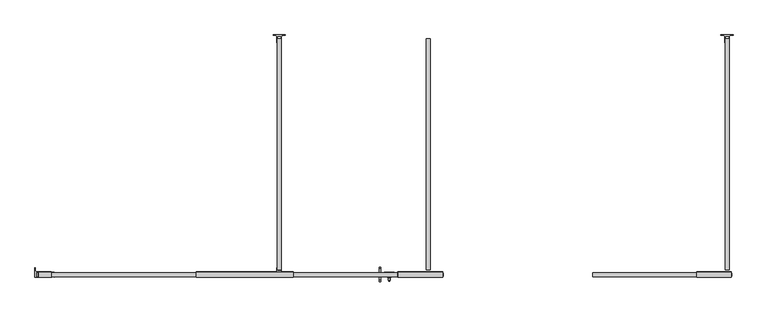
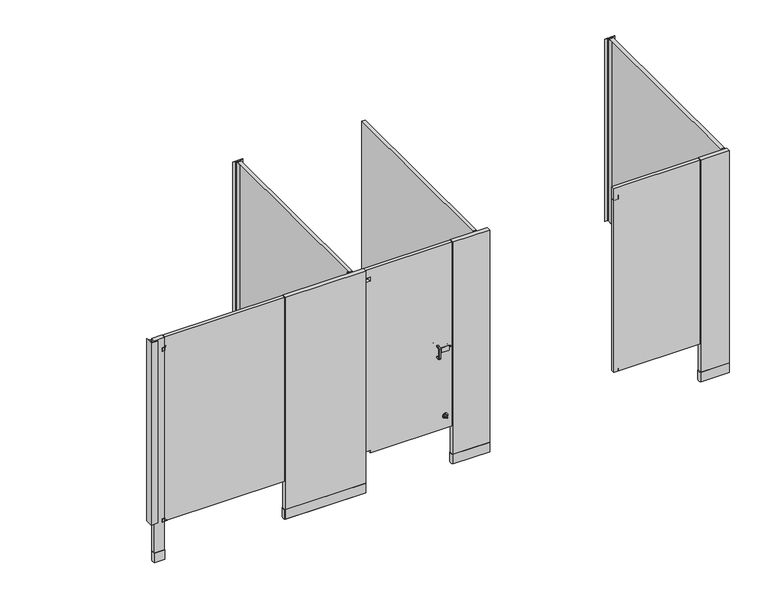
"""IFC4 building model written with IfcOpenShell, lengths in millimetres: proxy geometry, Partition-Floor_Braced-Bradley_Corp-St_Stl-ADA-N_Stalls : ADA (optional) + n Standard Stalls."""

from ifc_helpers import new_model, si_unit, point, frame, frame_2d, origin, origin_with_axes, place, context, project, spatial, polyline, circle_curve, ellipse_curve, trimmed, segment, composite_curve, outline, extrude, source, transform, mapped, element, save
from ifc_brep_helpers import plane_surface, cylinder_surface, revolved_surface, advanced_brep


def specialty_equipment_511efb68(model_context):
    return source(origin(), model_context, "Body", "SolidModel", [
        extrude(outline(composite_curve([segment(polyline([(4584.7002547, 3.175), (4584.7002547, 0.635), (4568.1902547, 0.635)]), True, "CONTINUOUS"), segment(trimmed(circle_curve(frame_2d((4568.1902547, -5.715)), 6.35), [point((4568.1902547, 0.635))], [point((4561.8402547, -5.715))], True, "CARTESIAN"), True, "CONTINUOUS"), segment(polyline([(4561.8402547, -5.715), (4561.8402547, -47.625), (4559.3002547, -47.625), (4559.3002547, -3.7728188), (4533.9002547, -3.7728188), (4533.9002547, -47.625), (4531.3602547, -47.625), (4531.3602547, -5.715)]), True, "CONTINUOUS"), segment(trimmed(circle_curve(frame_2d((4525.0102547, -5.715)), 6.35), [point((4531.3602547, -5.715))], [point((4525.0102547, 0.635))], True, "CARTESIAN"), True, "CONTINUOUS"), segment(polyline([(4525.0102547, 0.635), (4508.5002547, 0.635), (4508.5002547, 3.175), (4584.7002547, 3.175)]), True, "CONTINUOUS")], self_intersect=False)), frame((0.0, 0.0, 311.15), z_axis=(0.0, 0.0, 1.0), x_axis=(1.0, 0.0, 0.0)), (0.0, 0.0, 1.0), 1460.5),
        extrude(outline(composite_curve([segment(trimmed(circle_curve(frame_2d((301.9554547, -1504.95)), 2.54), [point((301.9554547, -1507.49))], [point((301.9554547, -1502.41))], False, "CARTESIAN"), True, "CONTINUOUS"), segment(trimmed(circle_curve(frame_2d((301.9554547, -1504.95)), 2.54), [point((301.9554547, -1502.41))], [point((301.9554547, -1507.49))], False, "CARTESIAN"), True, "CONTINUOUS")], self_intersect=False)), frame((0.0, 0.0, 304.8), z_axis=(0.0, 0.0, 1.0), x_axis=(1.0, 0.0, 0.0)), (0.0, 0.0, 1.0), 25.4),
        extrude(outline(composite_curve([segment(polyline([(292.1002547, -1489.71), (313.6902547, -1489.075), (323.8502547, -1497.33)]), True, "CONTINUOUS"), segment(trimmed(circle_curve(frame_2d((320.0402547, -1504.95)), 8.519419), [point((323.8502547, -1497.33))], [point((323.8502547, -1512.57))], False, "CARTESIAN"), True, "CONTINUOUS"), segment(polyline([(323.8502547, -1512.57), (313.6902547, -1520.825), (292.1002547, -1520.19), (292.1002547, -1489.71)]), True, "CONTINUOUS")], self_intersect=False)), frame((0.0, 0.0, 304.8), z_axis=(0.0, 0.0, 1.0), x_axis=(1.0, 0.0, 0.0)), (0.0, 0.0, 1.0), 3.81),
        extrude(outline(composite_curve([segment(polyline([(273.0502547, -1486.535), (292.1002547, -1486.535)]), True, "CONTINUOUS"), segment(trimmed(circle_curve(frame_2d((292.1002547, -1489.075)), 2.54), [point((292.1002547, -1486.535))], [point((294.6402547, -1489.075))], False, "CARTESIAN"), True, "CONTINUOUS"), segment(trimmed(circle_curve(frame_2d((186.8397496, -1504.95)), 108.9631338), [point((294.6402547, -1489.075))], [point((294.6402547, -1520.825))], False, "CARTESIAN"), True, "CONTINUOUS"), segment(trimmed(circle_curve(frame_2d((292.1002547, -1520.825)), 2.54), [point((294.6402547, -1520.825))], [point((292.1002547, -1523.365))], False, "CARTESIAN"), True, "CONTINUOUS"), segment(polyline([(292.1002547, -1523.365), (273.0502547, -1523.365), (273.0502547, -1486.535)]), True, "CONTINUOUS")], self_intersect=False)), frame((0.0, 0.0, 304.8), z_axis=(0.0, 0.0, 1.0), x_axis=(1.0, 0.0, 0.0)), (0.0, 0.0, 1.0), 25.4),
        extrude(outline(composite_curve([segment(trimmed(circle_curve(frame_2d((301.9554547, -1504.95)), 2.54), [point((301.9554547, -1507.49))], [point((301.9554547, -1502.41))], False, "CARTESIAN"), True, "CONTINUOUS"), segment(trimmed(circle_curve(frame_2d((301.9554547, -1504.95)), 2.54), [point((301.9554547, -1502.41))], [point((301.9554547, -1507.49))], False, "CARTESIAN"), True, "CONTINUOUS")], self_intersect=False)), frame((0.0, 0.0, 1676.4), z_axis=(0.0, 0.0, 1.0), x_axis=(1.0, 0.0, 0.0)), (0.0, 0.0, 1.0), 25.4),
        extrude(outline(composite_curve([segment(polyline([(296.8754547, -1520.825), (292.1002547, -1520.19), (292.1002547, -1489.71), (296.8754547, -1489.075), (307.0354547, -1497.33)]), True, "CONTINUOUS"), segment(trimmed(circle_curve(frame_2d((303.2254547, -1504.95)), 8.519419), [point((307.0354547, -1497.33))], [point((307.0354547, -1512.57))], False, "CARTESIAN"), True, "CONTINUOUS"), segment(polyline([(307.0354547, -1512.57), (296.8754547, -1520.825)]), True, "CONTINUOUS")], self_intersect=False)), frame((0.0, 0.0, 1697.99), z_axis=(0.0, 0.0, 1.0), x_axis=(1.0, 0.0, 0.0)), (0.0, 0.0, 1.0), 3.81),
        extrude(outline(composite_curve([segment(polyline([(273.0502547, -1486.535), (292.1002547, -1486.535)]), True, "CONTINUOUS"), segment(trimmed(circle_curve(frame_2d((292.1002547, -1489.075)), 2.54), [point((292.1002547, -1486.535))], [point((294.6402547, -1489.075))], False, "CARTESIAN"), True, "CONTINUOUS"), segment(trimmed(circle_curve(frame_2d((186.8397496, -1504.95)), 108.9631338), [point((294.6402547, -1489.075))], [point((294.6402547, -1520.825))], False, "CARTESIAN"), True, "CONTINUOUS"), segment(trimmed(circle_curve(frame_2d((292.1002547, -1520.825)), 2.54), [point((294.6402547, -1520.825))], [point((292.1002547, -1523.365))], False, "CARTESIAN"), True, "CONTINUOUS"), segment(polyline([(292.1002547, -1523.365), (273.0502547, -1523.365), (273.0502547, -1486.535)]), True, "CONTINUOUS")], self_intersect=False)), frame((0.0, 0.0, 1676.4), z_axis=(0.0, 0.0, 1.0), x_axis=(1.0, 0.0, 0.0)), (0.0, 0.0, 1.0), 25.4),
        extrude(outline(composite_curve([segment(polyline([(190.5002547, -1463.675), (193.0402547, -1463.675), (193.0402547, -1480.185)]), True, "CONTINUOUS"), segment(trimmed(circle_curve(frame_2d((199.3902547, -1480.185)), 6.35), [point((193.0402547, -1480.185))], [point((199.3902547, -1486.535))], True, "CARTESIAN"), True, "CONTINUOUS"), segment(polyline([(199.3902547, -1486.535), (241.3002547, -1486.535), (241.3002547, -1489.075), (197.4480735, -1489.075), (197.4480735, -1520.825), (241.3002547, -1520.825), (241.3002547, -1523.365), (190.5002547, -1523.365), (190.5002547, -1463.675)]), True, "CONTINUOUS")], self_intersect=False)), frame((0.0, 0.0, 311.15), z_axis=(0.0, 0.0, 1.0), x_axis=(1.0, 0.0, 0.0)), (0.0, 0.0, 1.0), 1460.5),
        extrude(outline(polyline([(1711.9602547, -1489.075), (1711.9602547, -1463.675), (1714.5002547, -1463.675), (1714.5002547, -1482.1271812), (1739.9002547, -1482.1271812), (1739.9002547, -1463.675), (1742.4402547, -1463.675), (1742.4402547, -1489.075), (1711.9602547, -1489.075)])), frame((0.0, 0.0, 311.15), z_axis=(0.0, 0.0, 1.0), x_axis=(1.0, 0.0, 0.0)), (0.0, 0.0, 1.0), 1460.5),
        extrude(outline(composite_curve([segment(polyline([(1765.3002547, 3.175), (1765.3002547, 0.635), (1748.7902547, 0.635)]), True, "CONTINUOUS"), segment(trimmed(circle_curve(frame_2d((1748.7902547, -5.715)), 6.35), [point((1748.7902547, 0.635))], [point((1742.4402547, -5.715))], True, "CARTESIAN"), True, "CONTINUOUS"), segment(polyline([(1742.4402547, -5.715), (1742.4402547, -47.625), (1739.9002547, -47.625), (1739.9002547, -3.7728188), (1714.5002547, -3.7728188), (1714.5002547, -47.625), (1711.9602547, -47.625), (1711.9602547, -5.715)]), True, "CONTINUOUS"), segment(trimmed(circle_curve(frame_2d((1705.6102547, -5.715)), 6.35), [point((1711.9602547, -5.715))], [point((1705.6102547, 0.635))], True, "CARTESIAN"), True, "CONTINUOUS"), segment(polyline([(1705.6102547, 0.635), (1689.1002547, 0.635), (1689.1002547, 3.175), (1765.3002547, 3.175)]), True, "CONTINUOUS")], self_intersect=False)), frame((0.0, 0.0, 311.15), z_axis=(0.0, 0.0, 1.0), x_axis=(1.0, 0.0, 0.0)), (0.0, 0.0, 1.0), 1460.5),
        extrude(outline(composite_curve([segment(polyline([(214.3127547, -1487.4875), (293.6891337, -1487.4875)]), True, "CONTINUOUS"), segment(trimmed(circle_curve(frame_2d((237.900102, -1504.95)), 58.4581471), [point((293.6891337, -1487.4875))], [point((293.6891337, -1522.4125))], False, "CARTESIAN"), True, "CONTINUOUS"), segment(polyline([(293.6891337, -1522.4125), (214.3127547, -1522.4125)]), True, "CONTINUOUS"), segment(trimmed(circle_curve(frame_2d((270.1017864, -1504.95)), 58.4581471), [point((214.3127547, -1522.4125))], [point((214.3127547, -1487.4875))], False, "CARTESIAN"), True, "CONTINUOUS")], self_intersect=False)), origin_with_axes(), (0.0, 0.0, 1.0), 76.2),
        extrude(outline(composite_curve([segment(polyline([(1204.9127547, -1487.4875), (1817.6891337, -1487.4875)]), True, "CONTINUOUS"), segment(trimmed(circle_curve(frame_2d((1761.900102, -1504.95)), 58.4581471), [point((1817.6891337, -1487.4875))], [point((1817.6891337, -1522.4125))], False, "CARTESIAN"), True, "CONTINUOUS"), segment(polyline([(1817.6891337, -1522.4125), (1204.9127547, -1522.4125)]), True, "CONTINUOUS"), segment(trimmed(circle_curve(frame_2d((1260.7017864, -1504.95)), 58.4581471), [point((1204.9127547, -1522.4125))], [point((1204.9127547, -1487.4875))], False, "CARTESIAN"), True, "CONTINUOUS")], self_intersect=False)), origin_with_axes(), (0.0, 0.0, 1.0), 76.2),
        extrude(outline(composite_curve([segment(polyline([(4354.5127547, -1487.4875), (4573.5891337, -1487.4875)]), True, "CONTINUOUS"), segment(trimmed(circle_curve(frame_2d((4517.800102, -1504.95)), 58.4581471), [point((4573.5891337, -1487.4875))], [point((4573.5891337, -1522.4125))], False, "CARTESIAN"), True, "CONTINUOUS"), segment(polyline([(4573.5891337, -1522.4125), (4354.5127547, -1522.4125)]), True, "CONTINUOUS"), segment(trimmed(circle_curve(frame_2d((4410.3017864, -1504.95)), 58.4581471), [point((4354.5127547, -1522.4125))], [point((4354.5127547, -1487.4875))], False, "CARTESIAN"), True, "CONTINUOUS")], self_intersect=False)), origin_with_axes(), (0.0, 0.0, 1.0), 76.2),
        extrude(outline(composite_curve([segment(trimmed(circle_curve(frame_2d((-1469.3891724, 977.9)), 10.16), [point((-1469.3891724, 988.06))], [point((-1459.2291724, 977.9))], False, "CARTESIAN"), True, "CONTINUOUS"), segment(polyline([(-1459.2291724, 977.9), (-1459.2291724, 901.7)]), True, "CONTINUOUS"), segment(trimmed(circle_curve(frame_2d((-1469.3891724, 901.7)), 10.16), [point((-1459.2291724, 901.7))], [point((-1469.3891724, 891.54))], False, "CARTESIAN"), True, "CONTINUOUS"), segment(polyline([(-1469.3891724, 891.54), (-1492.2491724, 891.54), (-1492.2491724, 901.7), (-1469.3891724, 901.7)]), True, "CONTINUOUS"), segment(trimmed(circle_curve(frame_2d((-1469.3891724, 904.24)), 2.54), [point((-1469.3891724, 901.7))], [point((-1466.8491724, 904.24))], True, "CARTESIAN"), True, "CONTINUOUS"), segment(polyline([(-1466.8491724, 904.24), (-1466.8491724, 975.36)]), True, "CONTINUOUS"), segment(trimmed(circle_curve(frame_2d((-1469.3891724, 975.36)), 2.54), [point((-1466.8491724, 975.36))], [point((-1469.3891724, 977.9))], True, "CARTESIAN"), True, "CONTINUOUS"), segment(polyline([(-1469.3891724, 977.9), (-1492.2491724, 977.9), (-1492.2491724, 988.06), (-1469.3891724, 988.06)]), True, "CONTINUOUS")], self_intersect=False)), frame((2356.5228738, 0.0, 0.0), z_axis=(1.0, 0.0, 0.0), x_axis=(0.0, 1.0, 0.0)), (0.0, 0.0, 1.0), 11.4113578),
        extrude(outline(composite_curve([segment(polyline([(-1540.51, 988.06), (-1517.65, 988.06), (-1517.65, 977.9), (-1540.51, 977.9)]), True, "CONTINUOUS"), segment(trimmed(circle_curve(frame_2d((-1540.51, 975.36)), 2.54), [point((-1540.51, 977.9))], [point((-1543.05, 975.36))], True, "CARTESIAN"), True, "CONTINUOUS"), segment(polyline([(-1543.05, 975.36), (-1543.05, 904.24)]), True, "CONTINUOUS"), segment(trimmed(circle_curve(frame_2d((-1540.51, 904.24)), 2.54), [point((-1543.05, 904.24))], [point((-1540.51, 901.7))], True, "CARTESIAN"), True, "CONTINUOUS"), segment(polyline([(-1540.51, 901.7), (-1517.65, 901.7), (-1517.65, 891.54), (-1540.51, 891.54)]), True, "CONTINUOUS"), segment(trimmed(circle_curve(frame_2d((-1540.51, 901.7)), 10.16), [point((-1540.51, 891.54))], [point((-1550.67, 901.7))], False, "CARTESIAN"), True, "CONTINUOUS"), segment(polyline([(-1550.67, 901.7), (-1550.67, 977.9)]), True, "CONTINUOUS"), segment(trimmed(circle_curve(frame_2d((-1540.51, 977.9)), 10.16), [point((-1550.67, 977.9))], [point((-1540.51, 988.06))], False, "CARTESIAN"), True, "CONTINUOUS")], self_intersect=False)), frame((2356.5228738, 0.0, 0.0), z_axis=(1.0, 0.0, 0.0), x_axis=(0.0, 1.0, 0.0)), (0.0, 0.0, 1.0), 11.4113578),
        extrude(outline(composite_curve([segment(trimmed(circle_curve(frame_2d((406.4, 2420.9250547)), 3.4532283), [point((402.9467717, 2420.9250547))], [point((409.8532283, 2420.9250547))], False, "CARTESIAN"), True, "CONTINUOUS"), segment(trimmed(circle_curve(frame_2d((406.4, 2420.9250547)), 3.4532283), [point((409.8532283, 2420.9250547))], [point((402.9467717, 2420.9250547))], False, "CARTESIAN"), True, "CONTINUOUS")], self_intersect=False)), frame((0.0, -1548.13, 0.0), z_axis=(0.0, 1.0, 0.0), x_axis=(0.0, 0.0, 1.0)), (0.0, 0.0, 1.0), 7.62),
        advanced_brep(
        [(2420.9250547, -1517.65, 406.4), (2401.8750547, -1517.65, 406.4), (2439.9750547, -1517.65, 406.4), (2426.0050547, -1540.51, 406.4), (2415.8450547, -1540.51, 406.4), (2420.9250547, -1540.51, 406.4), (2426.0050547, -1525.27, 406.4), (2415.8450547, -1525.27, 406.4), (2431.0850547, -1520.19, 406.4), (2410.7650547, -1520.19, 406.4), (2439.9750547, -1520.19, 406.4), (2401.8750547, -1520.19, 406.4)],
        [
            (0, 1),
            (1, 2, circle_curve(frame((2420.9250547, -1517.65, 406.4), z_axis=(0.0, 1.0, 0.0), x_axis=(-1.0, 0.0, 0.0)), 19.05)),
            (2, 0),
            (2, 1, circle_curve(frame((2420.9250547, -1517.65, 406.4), z_axis=(0.0, 1.0, 0.0), x_axis=(-1.0, 0.0, 0.0)), 19.05)),
            (3, 4, circle_curve(frame((2420.9250547, -1540.51, 406.4), z_axis=(0.0, -1.0, 0.0), x_axis=(-1.0, 0.0, 0.0)), 5.08)),
            (4, 5),
            (5, 3),
            (4, 3, circle_curve(frame((2420.9250547, -1540.51, 406.4), z_axis=(0.0, -1.0, 0.0), x_axis=(-1.0, 0.0, 0.0)), 5.08)),
            (6, 7, circle_curve(frame((2420.9250547, -1525.27, 406.4), z_axis=(0.0, -1.0, 0.0), x_axis=(-1.0, 0.0, 0.0)), 5.08)),
            (7, 4),
            (3, 6),
            (7, 6, circle_curve(frame((2420.9250547, -1525.27, 406.4), z_axis=(0.0, -1.0, 0.0), x_axis=(-1.0, 0.0, 0.0)), 5.08)),
            (8, 9, circle_curve(frame((2420.9250547, -1520.19, 406.4), z_axis=(0.0, -1.0, 0.0), x_axis=(-1.0, 0.0, 0.0)), 10.16)),
            (9, 7, circle_curve(frame((2415.8450547, -1520.19, 406.4), z_axis=(0.0, 0.0, 1.0), x_axis=(0.0, -1.0, 0.0)), 5.08)),
            (6, 8, circle_curve(frame((2426.0050547, -1520.19, 406.4), z_axis=(0.0, 0.0, 1.0), x_axis=(0.0, -1.0, 0.0)), 5.08)),
            (9, 8, circle_curve(frame((2420.9250547, -1520.19, 406.4), z_axis=(0.0, -1.0, 0.0), x_axis=(-1.0, 0.0, 0.0)), 10.16)),
            (10, 11, circle_curve(frame((2420.9250547, -1520.19, 406.4), z_axis=(0.0, -1.0, 0.0), x_axis=(-1.0, 0.0, 0.0)), 19.05)),
            (11, 9),
            (8, 10),
            (11, 10, circle_curve(frame((2420.9250547, -1520.19, 406.4), z_axis=(0.0, -1.0, 0.0), x_axis=(-1.0, 0.0, 0.0)), 19.05)),
            (1, 11),
            (10, 2),
        ],
        [
            plane_surface(frame((2420.9250547, -1517.65, 406.4), z_axis=(0.0, 1.0, 0.0), x_axis=(-1.0, 0.0, 0.0))),
            plane_surface(frame((2420.9250547, -1540.51, 406.4), z_axis=(0.0, -1.0, 0.0), x_axis=(-1.0, 0.0, 0.0))),
            cylinder_surface(frame((2420.9250547, -1561.6297247, 406.4), z_axis=(0.0, 1.0, 0.0), x_axis=(-1.0, 0.0, 0.0)), 5.08),
            revolved_surface(trimmed(ellipse_curve(frame((2415.8450547, -1520.19, 406.4), z_axis=(0.0, 0.0, -1.0), x_axis=(0.0, -1.0, 0.0)), 5.08, 5.08), [point((2415.8450547, -1525.27, 406.4))], [point((2410.7650547, -1520.19, 406.4))], True, "CARTESIAN"), (2420.9250547, -1561.6297247, 406.4), (0.0, 1.0, 0.0)),
            plane_surface(frame((2420.9250547, -1520.19, 406.4), z_axis=(0.0, -1.0, 0.0), x_axis=(-1.0, 0.0, 0.0))),
            cylinder_surface(frame((2420.9250547, -1561.6297247, 406.4), z_axis=(0.0, 1.0, 0.0), x_axis=(-1.0, 0.0, 0.0)), 19.05),
        ],
        [
            (0, [[1, 2, 3]]),
            (0, [[-3, 4, -1]]),
            (1, [[5, 6, 7]]),
            (1, [[8, -7, -6]]),
            (2, [[9, 10, -5, 11]]),
            (2, [[12, -11, -8, -10]]),
            (3, [[13, 14, -9, 15]]),
            (3, [[16, -15, -12, -14]]),
            (4, [[17, 18, -13, 19]]),
            (4, [[20, -19, -16, -18]]),
            (5, [[-2, 21, -17, 22]]),
            (5, [[-4, -22, -20, -21]]),
        ],
    ),
        advanced_brep(
        [(2465.3750547, -1499.87, 939.8), (2465.3750547, -1510.03, 939.8), (2482.8502547, -1510.03, 939.8), (2482.8502547, -1499.87, 939.8), (2465.3750547, -1504.95, 939.8), (2482.8502547, -1504.95, 939.8)],
        [
            (0, 1, circle_curve(frame((2465.3750547, -1504.95, 939.8), z_axis=(1.0, 0.0, 0.0), x_axis=(0.0, -1.0, 0.0)), 5.08)),
            (1, 2),
            (2, 3, circle_curve(frame((2482.8502547, -1504.95, 939.8), z_axis=(-1.0, 0.0, 0.0), x_axis=(0.0, -1.0, 0.0)), 5.08)),
            (3, 0),
            (1, 0, circle_curve(frame((2465.3750547, -1504.95, 939.8), z_axis=(1.0, 0.0, 0.0), x_axis=(0.0, -1.0, 0.0)), 5.08)),
            (3, 2, circle_curve(frame((2482.8502547, -1504.95, 939.8), z_axis=(-1.0, 0.0, 0.0), x_axis=(0.0, -1.0, 0.0)), 5.08)),
            (4, 1),
            (0, 4),
            (2, 5),
            (5, 3),
        ],
        [
            cylinder_surface(frame((2482.8502547, -1504.95, 939.8), z_axis=(-1.0, 0.0, 0.0), x_axis=(0.0, -1.0, 0.0)), 5.08),
            plane_surface(frame((2465.3750547, -1504.95, 939.8), z_axis=(-1.0, 0.0, 0.0), x_axis=(0.0, -1.0, 0.0))),
            plane_surface(frame((2482.8502547, -1504.95, 939.8), z_axis=(1.0, 0.0, 0.0), x_axis=(0.0, -1.0, 0.0))),
        ],
        [
            (0, [[1, 2, 3, 4]]),
            (0, [[5, -4, 6, -2]]),
            (1, [[7, -1, 8]]),
            (1, [[-8, -5, -7]]),
            (2, [[-3, 9, 10]]),
            (2, [[-6, -10, -9]]),
        ],
    ),
        extrude(outline(composite_curve([segment(trimmed(circle_curve(frame_2d((926.0058992, 2394.4309539)), 5.2558992), [point((926.0058992, 2389.1750547))], [point((920.75, 2394.4309539))], False, "CARTESIAN"), True, "CONTINUOUS"), segment(polyline([(920.75, 2394.4309539), (920.75, 2447.4191555)]), True, "CONTINUOUS"), segment(trimmed(circle_curve(frame_2d((926.0058992, 2447.4191555)), 5.2558992), [point((920.75, 2447.4191555))], [point((926.0058992, 2452.6750547))], False, "CARTESIAN"), True, "CONTINUOUS"), segment(polyline([(926.0058992, 2452.6750547), (953.5941008, 2452.6750547)]), True, "CONTINUOUS"), segment(trimmed(circle_curve(frame_2d((953.5941008, 2447.4191555)), 5.2558992), [point((953.5941008, 2452.6750547))], [point((958.85, 2447.4191555))], False, "CARTESIAN"), True, "CONTINUOUS"), segment(polyline([(958.85, 2447.4191555), (958.85, 2394.4309539)]), True, "CONTINUOUS"), segment(trimmed(circle_curve(frame_2d((953.5941008, 2394.4309539)), 5.2558992), [point((958.85, 2394.4309539))], [point((953.5941008, 2389.1750547))], False, "CARTESIAN"), True, "CONTINUOUS"), segment(polyline([(953.5941008, 2389.1750547), (926.0058992, 2389.1750547)]), True, "CONTINUOUS")], self_intersect=False)), frame((0.0, -1519.555, 0.0), z_axis=(0.0, 1.0, 0.0), x_axis=(0.0, 0.0, 1.0)), (0.0, 0.0, 1.0), 29.21),
        extrude(outline(composite_curve([segment(polyline([(2474.9127547, -1487.4875), (2757.4891337, -1487.4875)]), True, "CONTINUOUS"), segment(trimmed(circle_curve(frame_2d((2701.700102, -1504.95)), 58.4581471), [point((2757.4891337, -1487.4875))], [point((2757.4891337, -1522.4125))], False, "CARTESIAN"), True, "CONTINUOUS"), segment(polyline([(2757.4891337, -1522.4125), (2474.9127547, -1522.4125)]), True, "CONTINUOUS"), segment(trimmed(circle_curve(frame_2d((2530.7017864, -1504.95)), 58.4581471), [point((2474.9127547, -1522.4125))], [point((2474.9127547, -1487.4875))], False, "CARTESIAN"), True, "CONTINUOUS")], self_intersect=False)), origin_with_axes(), (0.0, 0.0, 1.0), 76.2),
        extrude(outline(polyline([(2679.7002547, -22.225), (2679.7002547, -1476.375), (2654.3002547, -1476.375), (2654.3002547, -22.225), (2679.7002547, -22.225)])), frame((0.0, 0.0, 304.8), z_axis=(0.0, 0.0, 1.0), x_axis=(1.0, 0.0, 0.0)), (0.0, 0.0, 1.0), 1473.2),
        extrude(outline(polyline([(2476.5002547, -1489.075), (2755.9002547, -1489.075), (2755.9002547, -1520.825), (2476.5002547, -1520.825), (2476.5002547, -1489.075)])), origin_with_axes(), (0.0, 0.0, 1.0), 1778.0),
        extrude(outline(polyline([(1778.0, 2471.7250547), (1778.0, 1820.8754547), (1714.5, 1820.8754547), (1714.5, 1852.6254547), (1682.75, 1852.6254547), (1682.75, 1820.8754547), (323.85, 1820.8754547), (323.85, 1852.6254547), (304.8, 1852.6254547), (304.8, 2471.7250547), (1778.0, 2471.7250547)])), frame((0.0, -1517.65, 0.0), z_axis=(0.0, 1.0, 0.0), x_axis=(0.0, 0.0, 1.0)), (0.0, 0.0, 1.0), 25.4),
        extrude(outline(polyline([(1201.7250547, -1517.65), (296.8754547, -1517.65), (296.8754547, -1492.25), (1201.7250547, -1492.25), (1201.7250547, -1517.65)])), frame((0.0, 0.0, 304.8), z_axis=(0.0, 0.0, 1.0), x_axis=(1.0, 0.0, 0.0)), (0.0, 0.0, 1.0), 1473.2),
        extrude(outline(polyline([(4351.3250547, -1517.65), (3700.4754547, -1517.65), (3700.4754547, -1492.25), (4351.3250547, -1492.25), (4351.3250547, -1517.65)])), frame((0.0, 0.0, 304.8), z_axis=(0.0, 0.0, 1.0), x_axis=(1.0, 0.0, 0.0)), (0.0, 0.0, 1.0), 1473.2),
        extrude(outline(polyline([(1778.0, 4351.3250547), (1778.0, 3700.4754547), (1714.5, 3700.4754547), (1714.5, 3732.2254547), (1682.75, 3732.2254547), (1682.75, 3700.4754547), (323.85, 3700.4754547), (323.85, 3732.2254547), (304.8, 3732.2254547), (304.8, 4351.3250547), (1778.0, 4351.3250547)])), frame((0.0, -1517.65, 0.0), z_axis=(0.0, 1.0, 0.0), x_axis=(0.0, 0.0, 1.0)), (0.0, 0.0, 1.0), 25.4),
        extrude(outline(polyline([(1778.0, 1201.7250547), (1778.0, 296.8754547), (1714.5, 296.8754547), (1714.5, 328.6254547), (1682.75, 328.6254547), (1682.75, 296.8754547), (323.85, 296.8754547), (323.85, 328.6254547), (304.8, 328.6254547), (304.8, 1201.7250547), (1778.0, 1201.7250547)])), frame((0.0, -1517.65, 0.0), z_axis=(0.0, 1.0, 0.0), x_axis=(0.0, 0.0, 1.0)), (0.0, 0.0, 1.0), 25.4),
        extrude(outline(polyline([(4356.1002547, -1489.075), (4572.0002547, -1489.075), (4572.0002547, -1520.825), (4356.1002547, -1520.825), (4356.1002547, -1489.075)])), origin_with_axes(), (0.0, 0.0, 1.0), 1778.0),
        extrude(outline(polyline([(1206.5002547, -1489.075), (1816.1002547, -1489.075), (1816.1002547, -1520.825), (1206.5002547, -1520.825), (1206.5002547, -1489.075)])), origin_with_axes(), (0.0, 0.0, 1.0), 1778.0),
        extrude(outline(polyline([(215.9002547, -1489.075), (292.1002547, -1489.075), (292.1002547, -1520.825), (215.9002547, -1520.825), (215.9002547, -1489.075)])), origin_with_axes(), (0.0, 0.0, 1.0), 1778.0),
        extrude(outline(polyline([(4533.9002547, -1476.375), (4533.9002547, -22.225), (4559.3002547, -22.225), (4559.3002547, -1476.375), (4533.9002547, -1476.375)])), frame((0.0, 0.0, 304.8), z_axis=(0.0, 0.0, 1.0), x_axis=(1.0, 0.0, 0.0)), (0.0, 0.0, 1.0), 1473.2),
        extrude(outline(polyline([(1714.5002547, -1476.375), (1714.5002547, -22.225), (1739.9002547, -22.225), (1739.9002547, -1476.375), (1714.5002547, -1476.375)])), frame((0.0, 0.0, 304.8), z_axis=(0.0, 0.0, 1.0), x_axis=(1.0, 0.0, 0.0)), (0.0, 0.0, 1.0), 1473.2),
    ])


if __name__ == "__main__":
    model = new_model("IFC4")
    model_context = context("Model", 3, world=origin())
    ifc_project = project(units=[si_unit("LENGTHUNIT", "METRE", prefix="MILLI")], contexts=[model_context])
    site = spatial("IfcSite", under=ifc_project)
    building = spatial("IfcBuilding", under=site)
    placement = place(None, origin())
    specialty_equipment_shape = specialty_equipment_511efb68(model_context)
    element("IfcBuildingElementProxy", 1, Name="Partition-Floor_Braced-Bradley_Corp-St_Stl-ADA-N_Stalls : ADA (optional) + n Standard Stalls", ObjectType="Partition-Floor_Braced-Bradley_Corp-St_Stl-ADA-N_Stalls : ADA (optional) + n Standard Stalls", at=placement, inside=building, context=model_context, shape_type="MappedRepresentation", body=[
        mapped(specialty_equipment_shape, transform((0.0, 0.0, 0.0), x_axis=(1.0, 0.0, 0.0), y_axis=(0.0, 1.0, 0.0), z_axis=(0.0, 0.0, 1.0))),
    ])
    save(model, "model.ifc")

# Revit data of these elements
# Type "Partition-Floor_Braced-Bradley_Corp-St_Stl-ADA-N_Stalls : ADA (optional) + n Standard Stalls"
#   Keynote = "M10211313.01"
#   Warranty Information = "Warranted 15 years against rust out, 5 years on chrome hardware, lifetime of the partition on the stainless steel hardware."
#   Version = "1.3"
#   URL = "http://www.bradleycorp.com/"
#   Type Comments = "n/a"
#   Technical Data = "n/a"
#   Keynote = "M10211313.01"
#   OmniClass Title = "Toilet Compartment and Urinal Screens"
#   OmniClass Code = "23.15.11.15.11"
#   Modeling Code = "n/a"
#   Model = "Stainless Steel - Series 500 - Floor Braced"
#   Material Note = "Other Hardware Also Available - Please See www.bradleycorp.com"
#   Material = "Metal - Bradley Corp - Chrome"
#   MasterFormat Title = "Toilet Compartments"
#   MasterFormat Number = "10 21 13"
#   Manufacturer = "Bradley Corporation"
#   LEED Credit = ""
#   Industry Standards = "n/a"
#   Fire Rating = "n/a"
#   Description = "Restroom Partitions, Floor-Braced"
#   Copyright = "This Model Data is Property of Bradley Corporation"
#   Complies to NAFTA = "n/a"
#   Buy American Act = "To Be Determined"
#   Assembly Code = "C1010400"
#   ADA Compliant [instance default] = "Yes"
#   Width [instance default] = 11' - 5"
#   Top Hinge = 5' - 7"
#   Door Opening Standard [instance default] = 2' - 2"
#   Door Opening Angle [instance default] = 0.00°
#   MaskR [instance default] = 3' - 1"
#   Mask M [instance default] = 3' - 1"
#   Mask [instance default] = 5' - 1"
#   Shoe Height = 0' - 3"
#   RPn [instance default] = 0' - 1"
#   Pilaster Height = 5' - 10"
#   Latch to Edge = 0' - 2"
#   Latch Height = 3' - 1"
#   LPn [instance default] = 0' - 1"
#   Start STDA [instance default] = 0' - 0"
#   Start STD [instance default] = 5' - 5 1/2"
#   Start AMB [instance default] = 0' - 4 1/2"
#   Start STD2 [instance default] = 8' - 6 1/2"
#   Stall Width Standard [instance default] = 3' - 0"
#   Stall Depth [instance default] = 4' - 10 3/4"
#   Right Pilaster Width STD [instance default] = 0' - 3"
#   Pilaster Thickness = 0' - 1 1/4"
#   Percentage of Recycled Content = 0
#   Panel Thickness = 0' - 1"
#   Left Pilaster Width [instance default] = 0' - 4 1/2"
#   Height = 5' - 10"
#   Gap Side Wall Right [instance default] = 0' - 0"
#   Gap Side Wall Left [instance default] = 0' - 0"
#   Gap Pilaster Panel = 0' - 0 1/2"
#   Gap Back Wall [instance default] = 0' - 1"
#   End Right Pilaster = 0' - 0 1/2"
#   Door Width Standard [instance default] = 2' - 1.624"
#   Door Width ADA [instance default] = 2' - 11.624"
#   Door Thickness = 0' - 1"
#   Door Swing Angle [instance default] = 0.00°
#   Door Opening ADA [instance default] = 3' - 0"
#   Door Height = 4' - 10"
#   Door Handle Height = 3' - 1"
#   Door Gap = 0' - 0.188"
#   Depth [instance default] = 5' - 0"
#   CALC_Start STDs [instance default] = 5' - 5 1/2"
#   CALC_WidthA [instance default] = 3' - 1"
#   CALC_STDA Width [instance default] = 0' - 5"
#   CALC_STD2 Width [instance default] = 2' - 9"
#   CALC_RP [instance default] = 0' - 0"
#   CALC_Half Pilaster = 0' - 0 5/8"
#   CALC_Half Door Width = 0' - 11"
#   CALC_STD1 Width [instance default] = 2' - 9"
#   CALC_Left [instance default] = 0' - 4 1/2"
#   CALC_Half Panel = 0' - 0 1/2"
#   CALC_Angle [instance default] = 30.00°
#   CALC_AMB Width [instance default] = 4' - 9"
#   CALC_ADAngle [instance default] = 0.00°
#   CALC_ADADoorW [instance default] = 2' - 11.624"
#   CALC_ADADoorSwing [instance default] = 0.00°
#   CALC_ADADiff [instance default] = 2' - 0"
#   Bumper Height = 1' - 4"
#   Bottom Hinge = 1' - 0"
#   Bottom AFF = 1' - 0"
#   Brackets Top Height = 5' - 4"
#   Brackets Bottom Height = 1' - 6"
#   Right Pilaster Width AMB [instance default] = 0' - 3"
#   Stall Width ADA [instance default] = 5' - 0"
#   Outswing Door ADA [instance default] = yes
#   Instructions On-Off Visibility = yes
#   Outswing Door [instance default] = no
#   STDA [instance default] = no
#   STD2 [instance default] = yes
#   STD1 [instance default] = yes
#   RP STD2 [instance default] = yes
#   RP STD1 [instance default] = yes
#   RP AMB [instance default] = yes
#   Stalls Array [instance default] = 2
#   Right Panel [instance default] = yes
#   Stalls [instance default] = 3
#   Left Panel [instance default] = yes
#   Continuous Brackets [instance default] = yes
#   CALC_STD2Out [instance default] = no
#   CALC_STD1Out [instance default] = no
#   CALC_OutADA [instance default] = yes
#   CALC_NSTD2Out [instance default] = yes
#   CALC_NSTD1Out [instance default] = yes
#   CALC_NRP [instance default] = no
#   CALC_NOutADA [instance default] = no
#   CALC_NLF [instance default] = no
#   CALC_ADAOut [instance default] = yes
#   Brackets [instance default] = no
#   ADA Stall [instance default] = yes
#   Shoe Material = Metal - Bradley Corp - Stainless Steel Satin
#   Hardware Material = Metal - Bradley Corp - Chrome
#   Partition Material = Metal - Bradley Corp - Chrome
# Element 1 (IfcBuildingElementProxy, "Partition-Floor_Braced-Bradley_Corp-St_Stl-ADA-N_Stalls : ADA (optional) + n Standard Stalls")
#   Width = 14' - 4 1/2"
#   Mask = 5' - 0 1/2"
#   LPn = 0' - 0"
#   Start STDA = 5' - 4"
#   Start STD = 0' - 0"
#   Start AMB = 0' - 4"
#   Start STD2 = 11' - 6"
#   Left Pilaster Width = 0' - 3"
#   Gap Side Wall Left = 0' - 1"
#   CALC_Start STDs = 5' - 4"
#   CALC_STDA Width = 2' - 9"
#   CALC_STD1 Width = 2' - 7 1/2"
#   CALC_Left = 0' - 4"
#   CALC_Angle = 0.00°
#   CALC_AMB Width = 4' - 8"
#   Outswing Door = yes
#   STDA = yes
#   STD1 = no
#   RP STD1 = no
#   Stalls = 4
#   Left Panel = no
#   CALC_STD2Out = yes
#   CALC_NSTD2Out = no
#   CALC_NSTD1Out = no
#   CALC_NLF = yes
#   Materials on its faces: "Metal - Bradley Corp - Chrome", "Metal - Bradley Corp - Stainless Steel Satin", "Plastic - Bradley Corp - Black"
# Materials
#   "Metal - Bradley Corp - Stainless Steel Satin": class "Metal", colour RGB 189 187 185, transparency 0
#   "Metal - Bradley Corp - Chrome": class "Metal", colour RGB 106 119 125, transparency 0, Cost = 0
#   "Plastic - Bradley Corp - Black": class "Plastic", colour RGB 5 5 5, transparency 0
